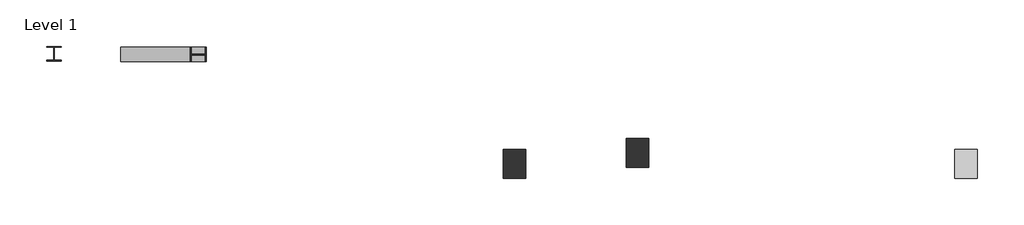
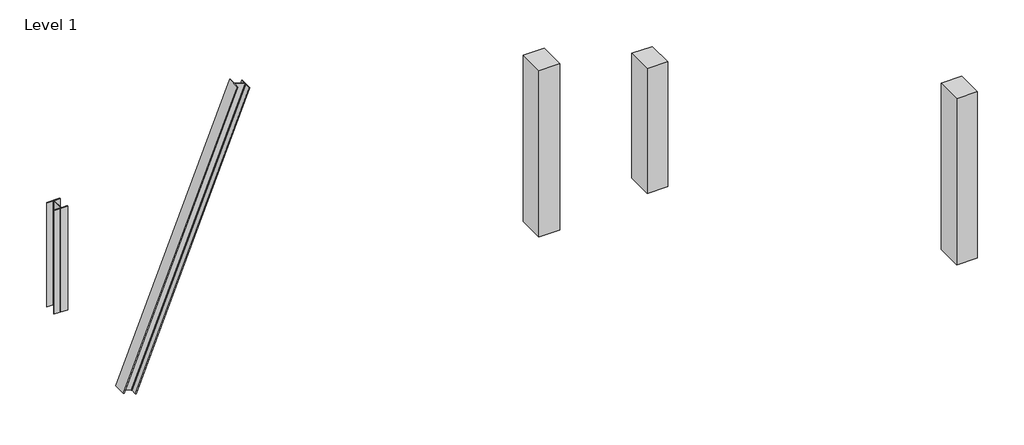
# One storey: 5 columns.
"""IFC4 building model written with IfcOpenShell, lengths in millimetres."""

import ifcopenshell
import ifcopenshell.guid

model = None  # the IFC model being written
_history = None  # IfcOwnerHistory: only IFC2X3 demands one
_inside = {}  # id of a spatial element -> (the spatial element, [elements in it])
_under = {}  # id of a project, library or spatial element -> (it, [spatial elements below it])
_declared = {}  # id of a project -> (the project, [libraries it declares])
_typed = {}  # id of a type object -> (the type object, [elements of that type])
_made_of = {}  # id of a material, layer set ... -> (it, [elements and type objects made of it])


def new_model(schema):
    """Start an empty IFC model of exactly this schema.

    Asked for "IFC4X3", IfcOpenShell would pick the latest addendum, in which some entities
    have other attributes; the version numbers below select the first issue.
    IFC2X3 requires an IfcOwnerHistory on every rooted entity: one is made here for all.
    """
    global model, _history
    if schema == "IFC4X3":
        model = ifcopenshell.file(schema_version=(4, 3, 0, 0))
    else:
        model = ifcopenshell.file(schema=schema)
    _inside.clear()
    _under.clear()
    _declared.clear()
    _typed.clear()
    _made_of.clear()
    _history = None
    if model.schema == "IFC2X3":
        org = make("IfcOrganization", Name="unknown")
        user = make(
            "IfcPersonAndOrganization",
            ThePerson=make("IfcPerson", FamilyName="unknown"),
            TheOrganization=org,
        )
        app = make(
            "IfcApplication",
            ApplicationDeveloper=org,
            Version="unknown",
            ApplicationFullName="unknown",
            ApplicationIdentifier="unknown",
        )
        _history = make(
            "IfcOwnerHistory",
            OwningUser=user,
            OwningApplication=app,
            ChangeAction="ADDED",
            CreationDate=0,
        )
    return model


def make(cls, **values):
    """One entity of the class cls with the attributes given. An attribute that is None is left unset."""
    return model.create_entity(
        cls, **{name: value for name, value in values.items() if value is not None}
    )


def rooted(cls, **values):
    """An entity with a GlobalId (a new one), such as an element, a storey or a relation."""
    return make(cls, GlobalId=ifcopenshell.guid.new(), OwnerHistory=_history, **values)


def si_unit(unit_type, name, prefix=None):
    """IfcSIUnit, for example si_unit("LENGTHUNIT", "METRE", prefix="MILLI")."""
    return make("IfcSIUnit", UnitType=unit_type, Prefix=prefix, Name=name)


def assignment(units):
    """IfcUnitAssignment: the units of a project."""
    return None if units is None else make("IfcUnitAssignment", Units=units)


def point(xyz):
    """IfcCartesianPoint."""
    return None if xyz is None else make("IfcCartesianPoint", Coordinates=xyz)


def direction(xyz):
    """IfcDirection."""
    return None if xyz is None else make("IfcDirection", DirectionRatios=xyz)


def frame(location, z_axis=None, x_axis=None):
    """IfcAxis2Placement3D, a coordinate frame: its origin and axes. An axis left out is left unset."""
    return make(
        "IfcAxis2Placement3D",
        Location=point(location),
        Axis=direction(z_axis),
        RefDirection=direction(x_axis),
    )


def frame_2d(location, x_axis=None):
    """IfcAxis2Placement2D, a coordinate frame in the plane: its origin and x axis."""
    return make(
        "IfcAxis2Placement2D", Location=point(location), RefDirection=direction(x_axis)
    )


def origin():
    """The frame at (0, 0, 0) with its axes left unset."""
    return frame((0.0, 0.0, 0.0))


def origin_with_axes():
    """The frame at (0, 0, 0) with the z axis (0, 0, 1) and the x axis (1, 0, 0) written out."""
    return frame((0.0, 0.0, 0.0), z_axis=(0.0, 0.0, 1.0), x_axis=(1.0, 0.0, 0.0))


def place(relative_to, where):
    """IfcLocalPlacement: puts the frame where relative to a parent placement (None: the world)."""
    return make(
        "IfcLocalPlacement", PlacementRelTo=relative_to, RelativePlacement=where
    )


def context(
    kind, dimensions, precision=None, world=None, true_north=None, identifier=None
):
    """IfcGeometricRepresentationContext, for example the 3D "Model" context."""
    return make(
        "IfcGeometricRepresentationContext",
        ContextIdentifier=identifier,
        ContextType=kind,
        CoordinateSpaceDimension=dimensions,
        Precision=precision,
        WorldCoordinateSystem=world,
        TrueNorth=true_north,
    )


def project(units=None, contexts=None):
    """IfcProject with its units and contexts."""
    return rooted(
        "IfcProject",
        Name="project",
        RepresentationContexts=contexts,
        UnitsInContext=assignment(units),
    )


def spatial(cls, under=None, at=None, **own):
    """A site, building, storey or space (cls), placed at a placement, below another one or the project."""
    s = rooted(cls, ObjectPlacement=at, **own)
    if under is not None:
        _under.setdefault(under.id(), (under, []))[1].append(s)
    return s


def polyline(points):
    """IfcPolyline through the points."""
    return make("IfcPolyline", Points=[point(p) for p in points])


def circle_curve(where, radius):
    """IfcCircle in the frame where."""
    return make("IfcCircle", Position=where, Radius=radius)


def trimmed(basis, trim1, trim2, sense, master):
    """IfcTrimmedCurve: the piece of a basis curve between two trims."""
    return make(
        "IfcTrimmedCurve",
        BasisCurve=basis,
        Trim1=trim1,
        Trim2=trim2,
        SenseAgreement=sense,
        MasterRepresentation=master,
    )


def segment(curve, same_sense, transition):
    """IfcCompositeCurveSegment."""
    return make(
        "IfcCompositeCurveSegment",
        Transition=transition,
        SameSense=same_sense,
        ParentCurve=curve,
    )


def composite_curve(segments, self_intersect=None):
    """IfcCompositeCurve: segments joined end to end."""
    return make("IfcCompositeCurve", Segments=segments, SelfIntersect=self_intersect)


def outline(outer, holes=None, kind="AREA"):
    """IfcArbitraryClosedProfileDef: a profile drawn as a closed curve; with holes, ...WithVoids."""
    if holes is None:
        return make("IfcArbitraryClosedProfileDef", ProfileType=kind, OuterCurve=outer)
    return make(
        "IfcArbitraryProfileDefWithVoids",
        ProfileType=kind,
        OuterCurve=outer,
        InnerCurves=holes,
    )


def extrude(swept, where, along, depth):
    """IfcExtrudedAreaSolid: the profile swept, set in the frame where, extruded along a direction by depth."""
    return make(
        "IfcExtrudedAreaSolid",
        SweptArea=swept,
        Position=where,
        ExtrudedDirection=direction(along),
        Depth=depth,
    )


def shape(context_of_items, identifier, shape_type, items):
    """IfcShapeRepresentation: the items that make up one representation, for example the "Body"."""
    return make(
        "IfcShapeRepresentation",
        ContextOfItems=context_of_items,
        RepresentationIdentifier=identifier,
        RepresentationType=shape_type,
        Items=items,
    )


def source(mapping_origin, context_of_items, identifier, shape_type, items):
    """IfcRepresentationMap: a shape defined once, which mapped items show again and again."""
    return make(
        "IfcRepresentationMap",
        MappingOrigin=mapping_origin,
        MappedRepresentation=shape(context_of_items, identifier, shape_type, items),
    )


def transform(
    local_origin,
    x_axis=None,
    y_axis=None,
    z_axis=None,
    scale=None,
    scale2=None,
    scale3=None,
    uniform=True,
):
    """IfcCartesianTransformationOperator3D, or its non-uniform kind. x_axis, y_axis, z_axis: its Axis1, 2, 3."""
    if uniform:
        return make(
            "IfcCartesianTransformationOperator3D",
            Axis1=direction(x_axis),
            Axis2=direction(y_axis),
            LocalOrigin=point(local_origin),
            Scale=scale,
            Axis3=direction(z_axis),
        )
    return make(
        "IfcCartesianTransformationOperator3DnonUniform",
        Axis1=direction(x_axis),
        Axis2=direction(y_axis),
        LocalOrigin=point(local_origin),
        Scale=scale,
        Axis3=direction(z_axis),
        Scale2=scale2,
        Scale3=scale3,
    )


def mapped(mapping_source, mapping_target):
    """IfcMappedItem: shows the shape of a source again, moved by a transform."""
    return make(
        "IfcMappedItem", MappingSource=mapping_source, MappingTarget=mapping_target
    )


def made_of(thing, what):
    """Note that an element or type object is made of a material, layer set ...; save() writes the relation."""
    if what is not None:
        _made_of.setdefault(what.id(), (what, []))[1].append(thing)
    return thing


def element(
    cls,
    number,
    at=None,
    inside=None,
    cuts=None,
    type_object=None,
    material=None,
    context=None,
    identifier="Body",
    shape_type=None,
    held_by="IfcProductDefinitionShape",
    body=None,
    shapes=None,
    **own,
):
    """One element of the class cls, such as IfcWall. Its Tag is "e" and its number.

    at: its placement. inside: the storey or other place that contains it. cuts: it is an
    opening in that element (IfcRelVoidsElement). A single representation is given by context,
    identifier, shape_type and body (its items); several are given by shapes. held_by: the class
    of the entity that holds the representations. save() writes the other relations.
    """
    e = rooted(cls, Tag="e%d" % number, ObjectPlacement=at, **own)
    if body is not None:
        shapes = [shape(context, identifier, shape_type, body)]
    if shapes is not None:
        e.Representation = make(held_by, Representations=shapes)
    if inside is not None:
        _inside.setdefault(inside.id(), (inside, []))[1].append(e)
    if cuts is not None:
        rooted(
            "IfcRelVoidsElement", RelatingBuildingElement=cuts, RelatedOpeningElement=e
        )
    if type_object is not None:
        _typed.setdefault(type_object.id(), (type_object, []))[1].append(e)
    return made_of(e, material)


def aggregate(whole, parts):
    """IfcRelAggregates: a whole, such as a stair, and the parts it consists of."""
    return rooted("IfcRelAggregates", RelatingObject=whole, RelatedObjects=parts)


def save(model, path):
    """Write the relations noted so far, then the file.

    IfcRelAggregates (storeys below a building ...), IfcRelContainedInSpatialStructure (elements
    in a storey), IfcRelDefinesByType, IfcRelAssociatesMaterial and IfcRelDeclares: one each for
    every whole, place, type object, material and project.
    """
    for whole, parts in _under.values():
        aggregate(whole, parts)
    for where, things in _inside.values():
        rooted(
            "IfcRelContainedInSpatialStructure",
            RelatedElements=things,
            RelatingStructure=where,
        )
    for kind, things in _typed.values():
        rooted("IfcRelDefinesByType", RelatedObjects=things, RelatingType=kind)
    for what, things in _made_of.values():
        rooted("IfcRelAssociatesMaterial", RelatedObjects=things, RelatingMaterial=what)
    for by, libraries in _declared.values():
        rooted("IfcRelDeclares", RelatingContext=by, RelatedDefinitions=libraries)
    model.write(path)


def m_rectangular_column_475_x_610mm_b7c60445(model_context):
    return source(origin(), model_context, "Body", "SweptSolid", [
        extrude(outline(polyline([(305.0, 237.5), (305.0, -237.5), (-305.0, -237.5), (-305.0, 237.5), (305.0, 237.5)])), origin_with_axes(), (0.0, 0.0, 1.0), 4000.0),
    ])


def m_rectangular_column_475_x_610mm_f11b4c06(model_context):
    return source(origin(), model_context, "Body", "SweptSolid", [
        extrude(outline(polyline([(305.0, 237.5), (305.0, -237.5), (-305.0, -237.5), (-305.0, 237.5), (305.0, 237.5)])), origin_with_axes(), (0.0, 0.0, 1.0), 3000.0),
    ])


def m_rectangular_column_475_x_610mm_1e9c0db0(model_context):
    return source(origin(), model_context, "Body", "SweptSolid", [
        extrude(outline(polyline([(305.0, 237.5), (305.0, -237.5), (-305.0, -237.5), (-305.0, 237.5), (305.0, 237.5)])), frame((0.0, 0.0, -4000.0), z_axis=(0.0, 0.0, 1.0), x_axis=(1.0, 0.0, 0.0)), (0.0, 0.0, 1.0), 4000.0),
    ])


def uc_universal_columns_column_uc305x305x97_3ae92ab7(model_context):
    return source(origin(), model_context, "Body", "SweptSolid", [
        extrude(outline(composite_curve([segment(polyline([(152.65, 153.95), (152.65, 138.55), (20.15, 138.55)]), True, "CONTINUOUS"), segment(trimmed(circle_curve(frame_2d((20.15, 123.35)), 15.2), [point((20.15, 138.55))], [point((4.95, 123.35))], True, "CARTESIAN"), True, "CONTINUOUS"), segment(polyline([(4.95, 123.35), (4.95, -123.35)]), True, "CONTINUOUS"), segment(trimmed(circle_curve(frame_2d((20.15, -123.35)), 15.2), [point((4.95, -123.35))], [point((20.15, -138.55))], True, "CARTESIAN"), True, "CONTINUOUS"), segment(polyline([(20.15, -138.55), (152.65, -138.55), (152.65, -153.95), (-152.65, -153.95), (-152.65, -138.55), (-20.15, -138.55)]), True, "CONTINUOUS"), segment(trimmed(circle_curve(frame_2d((-20.15, -123.35)), 15.2), [point((-20.15, -138.55))], [point((-4.95, -123.35))], True, "CARTESIAN"), True, "CONTINUOUS"), segment(polyline([(-4.95, -123.35), (-4.95, 123.35)]), True, "CONTINUOUS"), segment(trimmed(circle_curve(frame_2d((-20.15, 123.35)), 15.2), [point((-4.95, 123.35))], [point((-20.15, 138.55))], True, "CARTESIAN"), True, "CONTINUOUS"), segment(polyline([(-20.15, 138.55), (-152.65, 138.55), (-152.65, 153.95), (152.65, 153.95)]), True, "CONTINUOUS")], self_intersect=False)), origin_with_axes(), (0.0, 0.0, 1.0), 2500.0),
    ])


model = new_model("IFC4")

# Units and contexts
model_context = context("Model", 3, world=origin())
ifc_project = project(units=[si_unit("LENGTHUNIT", "METRE", prefix="MILLI")], contexts=[model_context])

# Site, building, storey
site = spatial("IfcSite", under=ifc_project)
building = spatial("IfcBuilding", under=site)
storey = spatial("IfcBuildingStorey", under=building, Name="Level 1", Elevation=0.0)

# Columns
placement = place(None, origin())
m_rectangular_column_475_x_610mm_shape = m_rectangular_column_475_x_610mm_b7c60445(model_context)
element("IfcColumn", 1, ObjectType="M_Rectangular Column : 475 x 610mm", at=placement, inside=storey, context=model_context, shape_type="MappedRepresentation", body=[
    mapped(m_rectangular_column_475_x_610mm_shape, transform((-6672.9984463, 10294.8525449, 0.0), x_axis=(0.0, 1.0, 0.0), y_axis=(-1.0, 0.0, 0.0), z_axis=(0.0, 0.0, 1.0))),
])
m_rectangular_column_475_x_610mm_2_shape = m_rectangular_column_475_x_610mm_f11b4c06(model_context)
element("IfcColumn", 2, ObjectType="M_Rectangular Column : 475 x 610mm", at=placement, inside=storey, context=model_context, shape_type="MappedRepresentation", body=[
    mapped(m_rectangular_column_475_x_610mm_2_shape, transform((-4082.8922313, 10521.457476, 0.0), x_axis=(0.0, 1.0, 0.0), y_axis=(-1.0, 0.0, 0.0), z_axis=(0.0, 0.0, 1.0))),
])
m_rectangular_column_475_x_610mm_3_shape = m_rectangular_column_475_x_610mm_1e9c0db0(model_context)
element("IfcColumn", 3, ObjectType="M_Rectangular Column : 475 x 610mm", at=placement, inside=storey, context=model_context, shape_type="MappedRepresentation", body=[
    mapped(m_rectangular_column_475_x_610mm_3_shape, transform((2827.0015537, 10294.8525449, 0.0), x_axis=(0.0, 1.0, 0.0), y_axis=(-1.0, 0.0, 0.0), z_axis=(0.0, 0.0, 1.0))),
])
element("IfcColumn", 4, ObjectType="UC-Universal Columns-Column : UC305x305x97", at=placement, inside=storey, context=model_context, shape_type="SweptSolid", body=[
    extrude(outline(composite_curve([segment(polyline([(305.3, 0.0), (305.3, -15.4), (172.8, -15.4)]), True, "CONTINUOUS"), segment(trimmed(circle_curve(frame_2d((172.8, -30.6)), 15.2), [point((172.8, -15.4))], [point((157.6, -30.6))], True, "CARTESIAN"), True, "CONTINUOUS"), segment(polyline([(157.6, -30.6), (157.6, -277.3)]), True, "CONTINUOUS"), segment(trimmed(circle_curve(frame_2d((172.8, -277.3)), 15.2), [point((157.6, -277.3))], [point((172.8, -292.5))], True, "CARTESIAN"), True, "CONTINUOUS"), segment(polyline([(172.8, -292.5), (305.3, -292.5), (305.3, -307.9), (0.0, -307.9), (0.0, -292.5), (132.5, -292.5)]), True, "CONTINUOUS"), segment(trimmed(circle_curve(frame_2d((132.5, -277.3)), 15.2), [point((132.5, -292.5))], [point((147.7, -277.3))], True, "CARTESIAN"), True, "CONTINUOUS"), segment(polyline([(147.7, -277.3), (147.7, -30.6)]), True, "CONTINUOUS"), segment(trimmed(circle_curve(frame_2d((132.5, -30.6)), 15.2), [point((147.7, -30.6))], [point((132.5, -15.4))], True, "CARTESIAN"), True, "CONTINUOUS"), segment(polyline([(132.5, -15.4), (0.0, -15.4), (0.0, 0.0), (305.3, 0.0)]), True, "CONTINUOUS")], self_intersect=False)), frame((-14945.4439574, 12442.2025449, -2442.7454711), z_axis=(0.37190340329626154, 0.0, 0.9282714358508821), x_axis=(0.0, 1.0, 0.0)), (0.0, 0.0, 1.0), 6965.1601637),
])
uc_universal_columns_column_uc305x305x97_shape = uc_universal_columns_column_uc305x305x97_3ae92ab7(model_context)
element("IfcColumn", 5, ObjectType="UC-Universal Columns-Column : UC305x305x97", at=placement, inside=storey, context=model_context, shape_type="MappedRepresentation", body=[
    mapped(uc_universal_columns_column_uc305x305x97_shape, transform((-16355.4655243, 12612.2564061, 0.0), x_axis=(1.0, 0.0, 0.0), y_axis=(0.0, 1.0, 0.0), z_axis=(0.0, 0.0, 1.0))),
])

save(model, "model.ifc")

# Revit data of these elements
# Project information
#   Project Issue Date = "Issue Date"
#   Project Status = "Project Status"
#   Client Name = "Owner"
#   Project Address = "Enter address here"
#   Project Name = "Project Name"
#   Project Number = "0001"
# Type "M_Rectangular Column : 475 x 610mm"
#   Depth = 475 mm
#   Offset Base = 0 mm
#   Offset Top = 0 mm
#   Width = 610 mm
#   Material = Copper
# Type "UC-Universal Columns-Column : UC305x305x97"
#   Section Name Key = "UC305x305x97"
#   Width = 30.53 cm
#   Web Thickness = 0.99 cm
#   Web Fillet = 1.52 cm
#   Warping Constant = 1560000.0 cm⁶
#   Torsional Moment of Inertia = 91.20 cm⁴
#   Section Area = 123.0 cm²
#   Plastic Modulus weak axis = 726.0 cm³
#   Plastic Modulus strong axis = 1592.0 cm³
#   Nominal Weight = 96.8996 kgf/m
#   Moment of Inertia weak axis = 7308.00 cm⁴
#   Moment of Inertia strong axis = 22249.00 cm⁴
#   Height = 30.79 cm
#   Flange Thickness = 1.54 cm
#   Elastic Modulus weak axis = 479.0 cm³
#   Elastic Modulus strong axis = 1445.0 cm³
#   Centroid Vertical = 15.395 cm
#   Centroid Horizontal = 15.265 cm
#   Bolt Spacing = 14.0 cm
#   Structural Material [instance default] = Metal - Steel 43-275
#   Type Comments = ""
#   Assembly Code = ""
# Element 1 (IfcColumn, "M_Rectangular Column : 475 x 610mm")
#   SpeckleObjectUpdateDescription = "No changes yet"
#   SpeckleObjectTestNumber = 6
#   Phase Created = New Construction
#   Materials on its faces: "Copper"
# Element 2 (IfcColumn, "M_Rectangular Column : 475 x 610mm")
#   SpeckleObjectUpdateDescription = "No changes yet"
#   SpeckleObjectTestNumber = 7
#   Phase Created = New Construction
#   Materials on its faces: "Copper"
# Element 3 (IfcColumn, "M_Rectangular Column : 475 x 610mm")
#   SpeckleObjectUpdateDescription = "No changes yet"
#   SpeckleObjectTestNumber = 9
#   Phase Created = New Construction
#   Materials on its faces: "Copper"
# Element 4 (IfcColumn, "UC-Universal Columns-Column : UC305x305x97")
#   SpeckleObjectUpdateDescription = "drag single end"
#   SpeckleObjectTestNumber = 3
#   Structural Material = Metal - Steel 43-275
#   Phase Created = New Construction
#   Materials on its faces: "Metal - Steel 43-275"
# Element 5 (IfcColumn, "UC-Universal Columns-Column : UC305x305x97")
#   SpeckleObjectUpdateDescription = "move column up"
#   SpeckleObjectTestNumber = 2
#   Structural Material = Metal - Steel 43-275
#   Phase Created = New Construction
#   Materials on its faces: "Metal - Steel 43-275"
# Materials
#   "Copper": class "Metal", colour RGB 0 0 0, transparency 0, Description = "Copper, matte finish", Cost = 0
#   "Metal - Steel 43-275": class "Metal", colour RGB 247 247 247, transparency 0, Cost = 0
